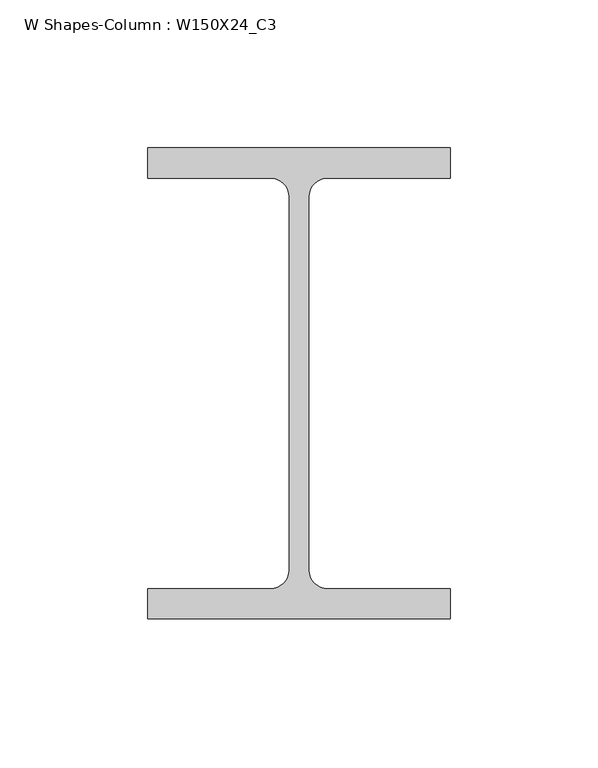
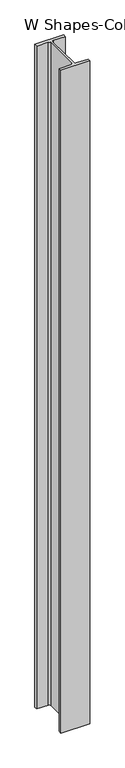
"""IFC4 building model written with IfcOpenShell, lengths in millimetres: column geometry, W Shapes-Column : W150X24_C3."""

from ifc_helpers import new_model, si_unit, point, frame, frame_2d, origin, place, context, project, spatial, polyline, circle_curve, trimmed, segment, composite_curve, outline, extrude, source, transform, mapped, element, save


def w_shapes_column_w150x24_c3_40a85f37(model_context):
    return source(origin(), model_context, "Body", "SweptSolid", [
        extrude(outline(composite_curve([segment(polyline([(51.181, 79.756), (51.181, 69.469), (9.652, 69.469)]), True, "CONTINUOUS"), segment(trimmed(circle_curve(frame_2d((9.652, 63.119)), 6.35), [point((9.652, 69.469))], [point((3.302, 63.119))], True, "CARTESIAN"), True, "CONTINUOUS"), segment(polyline([(3.302, 63.119), (3.302, -63.119)]), True, "CONTINUOUS"), segment(trimmed(circle_curve(frame_2d((9.652, -63.119)), 6.35), [point((3.302, -63.119))], [point((9.652, -69.469))], True, "CARTESIAN"), True, "CONTINUOUS"), segment(polyline([(9.652, -69.469), (51.181, -69.469), (51.181, -79.756), (-51.181, -79.756), (-51.181, -69.469), (-9.652, -69.469)]), True, "CONTINUOUS"), segment(trimmed(circle_curve(frame_2d((-9.652, -63.119)), 6.35), [point((-9.652, -69.469))], [point((-3.302, -63.119))], True, "CARTESIAN"), True, "CONTINUOUS"), segment(polyline([(-3.302, -63.119), (-3.302, 63.119)]), True, "CONTINUOUS"), segment(trimmed(circle_curve(frame_2d((-9.652, 63.119)), 6.35), [point((-3.302, 63.119))], [point((-9.652, 69.469))], True, "CARTESIAN"), True, "CONTINUOUS"), segment(polyline([(-9.652, 69.469), (-51.181, 69.469), (-51.181, 79.756), (51.181, 79.756)]), True, "CONTINUOUS")], self_intersect=False)), frame((0.0, 0.0, 506.0), z_axis=(0.0, 0.0, 1.0), x_axis=(1.0, 0.0, 0.0)), (0.0, 0.0, 1.0), 2484.0),
    ])


if __name__ == "__main__":
    model = new_model("IFC4")
    model_context = context("Model", 3, world=origin())
    ifc_project = project(units=[si_unit("LENGTHUNIT", "METRE", prefix="MILLI")], contexts=[model_context])
    site = spatial("IfcSite", under=ifc_project)
    building = spatial("IfcBuilding", under=site)
    placement = place(None, origin())
    w_shapes_column_w150x24_c3_shape = w_shapes_column_w150x24_c3_40a85f37(model_context)
    element("IfcColumn", 1, ObjectType="W Shapes-Column : W150X24_C3", at=placement, inside=building, context=model_context, shape_type="MappedRepresentation", body=[
        mapped(w_shapes_column_w150x24_c3_shape, transform((0.0, 0.0, 0.0), x_axis=(1.0, 0.0, 0.0), y_axis=(0.0, 1.0, 0.0), z_axis=(0.0, 0.0, 1.0))),
    ])
    save(model, "model.ifc")

# Revit data of these elements
# Type "W Shapes-Column : W150X24_C3"
#   Section Name Key = "W6x16"
#   Assembly Code = "B10"
#   Width = 10.2362 cm
#   Web Thickness = 0.6604 cm
#   Web Fillet = 0.635 cm
#   Warping Constant = 10258.1 cm⁶
#   Torsional Moment of Inertia = 9.28196 cm⁴
#   Section Area = 30.5806 cm²
#   Plastic Modulus weak axis = 55.5521 cm³
#   Plastic Modulus strong axis = 191.729 cm³
#   Perimeter = 0.704088 m²/m
#   Nominal Weight = 23.8106 kgf/m
#   Moment of Inertia weak axis = 184.391 cm⁴
#   Moment of Inertia strong axis = 1336.10 cm⁴
#   Height = 15.9512 cm
#   Flange Thickness = 1.0287 cm
#   Elastic Modulus weak axis = 36.0515 cm³
#   Elastic Modulus strong axis = 167.148 cm³
#   Clear Web Height = 19.05 cm
#   Centroid Vertical = 7.9756 cm
#   Centroid Horizontal = 5.1181 cm
#   Bolt Spacing = 5.715 cm
#   Structural Material [instance default] = Steel ASTM A992
#   Principal Axes Angle = 0
# Element 1 (IfcColumn, "W Shapes-Column : W150X24_C3")
#   Structural Material = none
# Materials
#   "Steel ASTM A992": class "Metal", colour RGB 199 199 199, transparency 0, Description = "Structural steel 50ksi", Cost = 0
